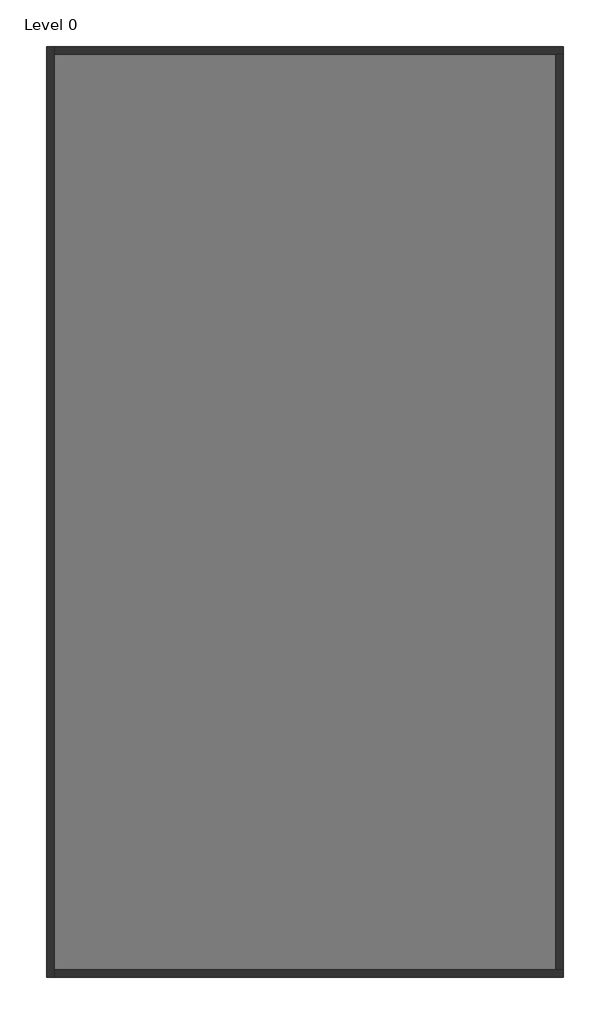
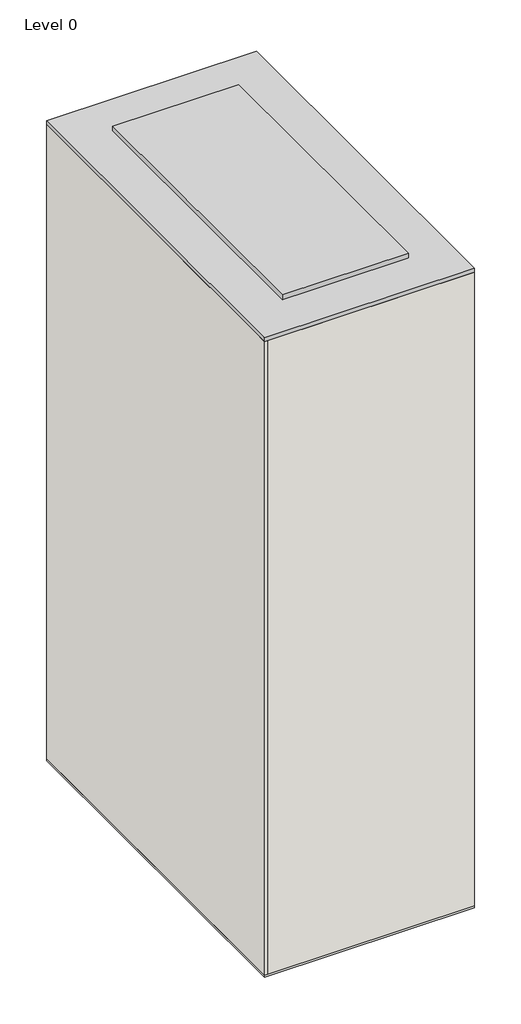
# One storey: 4 walls, 1 proxy, 1 slab.
"""IFC4 building model written with IfcOpenShell, lengths in millimetres."""

from ifc_helpers import new_model, si_unit, frame, origin, origin_with_axes, place, context, project, spatial, polyline, outline, extrude, faceted_brep, element, save

model = new_model("IFC4")

# Units and contexts
model_context = context("Model", 3, world=origin())
ifc_project = project(units=[si_unit("LENGTHUNIT", "METRE", prefix="MILLI")], contexts=[model_context])

# Site, building, storey
site = spatial("IfcSite", under=ifc_project)
building = spatial("IfcBuilding", under=site)
storey = spatial("IfcBuildingStorey", under=building, Name="Level 0", Elevation=100.0)

# Proxy
placement = place(None, origin())
element("IfcBuildingElementProxy", 1, Name="LowUrbanDensityBuilding : LowUrbanDensityBuilding", ObjectType="LowUrbanDensityBuilding : LowUrbanDensityBuilding", at=placement, inside=storey, context=model_context, shape_type="SweptSolid", body=[
    extrude(outline(polyline([(7325.2659446, 3676.2074539), (7325.2659446, -14323.7925461), (-2674.7340554, -14323.7925461), (-2674.7340554, 3676.2074539), (7325.2659446, 3676.2074539)])), origin_with_axes(), (0.0, 0.0, 1.0), 32200.0),
    extrude(outline(polyline([(5325.2659446, 1676.2074539), (5325.2659446, -12323.7925461), (-674.7340554, -12323.7925461), (-674.7340554, 1676.2074539), (5325.2659446, 1676.2074539)])), frame((0.0, 0.0, 32200.0), z_axis=(0.0, 0.0, 1.0), x_axis=(1.0, 0.0, 0.0)), (0.0, 0.0, 1.0), 245.0),
])

# Slab
element("IfcSlab", 2, ObjectType="Floor-Concrete_100Con", at=placement, inside=storey, context=model_context, shape_type="SweptSolid", body=[
    extrude(outline(polyline([(7325.2659446, 3676.2074539), (7325.2659446, -14323.7925461), (-2674.7340554, -14323.7925461), (-2674.7340554, 3676.2074539), (7325.2659446, 3676.2074539)])), origin_with_axes(), (0.0, 0.0, 1.0), 100.0),
])

# Walls
element("IfcWall", 3, ObjectType="Wall-Ext_25Rdr-100Blk-19P", at=placement, inside=storey, context=model_context, shape_type="Brep", body=[
    faceted_brep([(-2674.7340554, 3676.2074539, 100.0), (-2674.7340554, -14323.7925461, 100.0), (-2674.7340554, -14323.7925461, 32000.0), (-2674.7340554, 3676.2074539, 32000.0), (-2530.4340554, 3676.2074539, 100.0), (-2530.4340554, 3676.2074539, 32000.0), (-2530.4340554, 3531.9074539, 32000.0), (-2530.4340554, -14179.4925461, 32000.0), (-2530.4340554, -14323.7925461, 32000.0), (-2530.4340554, -14323.7925461, 100.0), (-2530.4340554, -14179.4925461, 100.0), (-2530.4340554, 3531.9074539, 100.0)], [[[0, 1, 2, 3]], [[4, 5, 6, 7, 8, 9, 10, 11]], [[1, 0, 4, 11, 10, 9]], [[3, 2, 8, 7, 6, 5]], [[2, 1, 9, 8]], [[0, 3, 5, 4]]]),
])
element("IfcWall", 4, ObjectType="Wall-Ext_25Rdr-100Blk-19P", at=placement, inside=storey, context=model_context, shape_type="Brep", body=[
    faceted_brep([(-2530.4340554, -14323.7925461, 100.0), (7325.2659446, -14323.7925461, 100.0), (7325.2659446, -14323.7925461, 32000.0), (-2530.4340554, -14323.7925461, 32000.0), (-2530.4340554, -14179.4925461, 100.0), (-2530.4340554, -14179.4925461, 32000.0), (7180.9659446, -14179.4925461, 32000.0), (7325.2659446, -14179.4925461, 32000.0), (7325.2659446, -14179.4925461, 100.0), (7180.9659446, -14179.4925461, 100.0)], [[[0, 1, 2, 3]], [[4, 5, 6, 7, 8, 9]], [[1, 0, 4, 9, 8]], [[3, 2, 7, 6, 5]], [[0, 3, 5, 4]], [[2, 1, 8, 7]]]),
])
element("IfcWall", 5, ObjectType="Wall-Ext_25Rdr-100Blk-19P", at=placement, inside=storey, context=model_context, shape_type="Brep", body=[
    faceted_brep([(7325.2659446, 3676.2074539, 100.0), (-2530.4340554, 3676.2074539, 100.0), (-2530.4340554, 3676.2074539, 32000.0), (7325.2659446, 3676.2074539, 32000.0), (7325.2659446, 3531.9074539, 100.0), (7325.2659446, 3531.9074539, 32000.0), (7180.9659446, 3531.9074539, 32000.0), (-2530.4340554, 3531.9074539, 32000.0), (-2530.4340554, 3531.9074539, 100.0), (7180.9659446, 3531.9074539, 100.0)], [[[0, 1, 2, 3]], [[4, 5, 6, 7, 8, 9]], [[1, 0, 4, 9, 8]], [[3, 2, 7, 6, 5]], [[2, 1, 8, 7]], [[0, 3, 5, 4]]]),
])
element("IfcWall", 6, ObjectType="Wall-Ext_25Rdr-100Blk-19P", at=placement, inside=storey, context=model_context, shape_type="SweptSolid", body=[
    extrude(outline(polyline([(7325.2659446, 3531.9074539), (7325.2659446, -14179.4925461), (7180.9659446, -14179.4925461), (7180.9659446, 3531.9074539), (7325.2659446, 3531.9074539)])), frame((0.0, 0.0, 100.0), z_axis=(0.0, 0.0, 1.0), x_axis=(1.0, 0.0, 0.0)), (0.0, 0.0, 1.0), 31900.0),
])

save(model, "model.ifc")

# Revit data of these elements
# Project information
#   Project Issue Date = "Issue Date"
#   Project Status = "Project Status"
#   Client Name = "Owner"
#   Project Address = "Enter address here"
#   Project Name = "Project Name"
#   Project Number = "Project Number"
# Type "Floor-Concrete_100Con"
#   Keynote = "E60/130"
#   Function = 0
#   Layers, outside or top first: 100 mm "Concrete" (function 1)
# Type "Wall-Ext_25Rdr-100Blk-19P"
#   Keynote = "F10"
#   Layers, outside or top first: 25.3 mm "Render, Beige, Smooth" (function 5); 100 mm "Concrete Masonry Units _Low Density" (function 1); 19 mm "Plaster" (function 5)
# Element 1 (IfcBuildingElementProxy, "LowUrbanDensityBuilding : LowUrbanDensityBuilding")
#   Phase Created = New Construction
#   Materials on its faces: "Default Form"
# Element 2 (IfcSlab, "Floor-Concrete_100Con")
#   Height Offset From Level = 0 mm
#   Phase Created = New Construction
#   Materials on its faces: "Concrete"
# Element 3 (IfcWall, "Wall-Ext_25Rdr-100Blk-19P")
#   Top Offset = 0 mm
#   Base Offset = 0 mm
#   wall height = 31900 mm
#   Phase Created = New Construction
#   Base Constraint = Level 0
#   Top Constraint = Level 8
#   Materials on its faces: "Render, Beige, Smooth", "Default Wall", "Plaster"
# Elements 4, 5, 6 (IfcWall, "Wall-Ext_25Rdr-100Blk-19P")
#   Top Offset = 0 mm
#   Base Offset = 0 mm
#   wall height = 31900 mm
#   Phase Created = New Construction
#   Base Constraint = Level 0
#   Top Constraint = Level 8
#   Materials on its faces: "Default Wall", "Render, Beige, Smooth", "Plaster"
# Materials
#   "Concrete": class "Concrete", colour RGB 120 120 120, transparency 0, Description = "Portland Cement Concrete", Cost = 0
#   "Render, Beige, Smooth": class "Generic", colour RGB 213 198 180, transparency 0, Description = "physical material", Cost = 0
#   "Concrete Masonry Units _Low Density": class "Masonry", colour RGB 181 181 181, transparency 0, Description = "Concrete masonry units", Cost = 0
#   "Plaster": class "Generic", colour RGB 249 249 249, transparency 0, Description = "Plaster", Cost = 0
#   "Default Form": class "Generic", colour RGB 185 189 196, transparency 0.5, Cost = 0
#   "Default Wall": class "Miscellaneous", colour RGB 128 128 128, transparency 0, Comments = "Rendering appearance not upgraded Rendering appearance not upgraded ", Cost = 0
